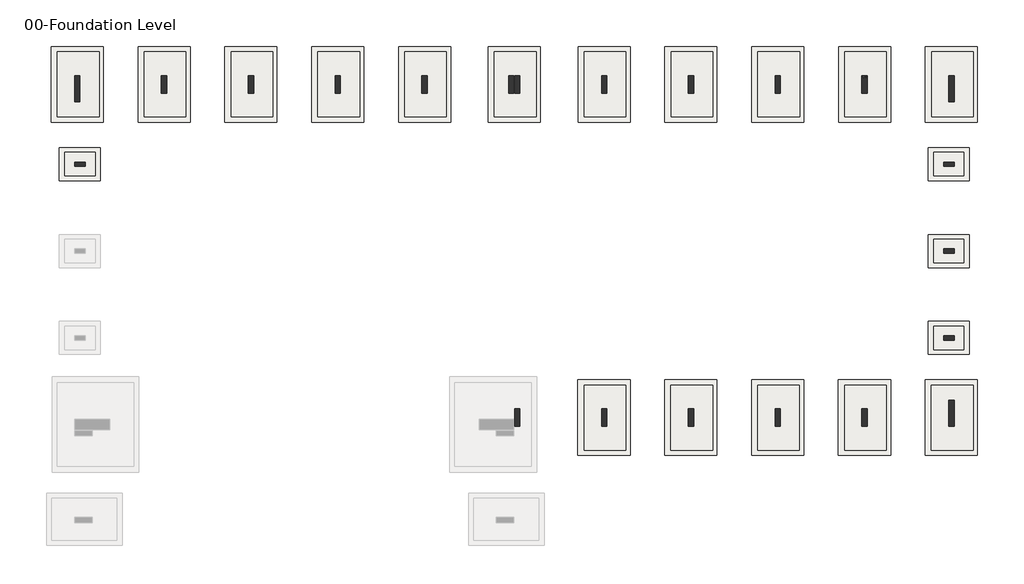
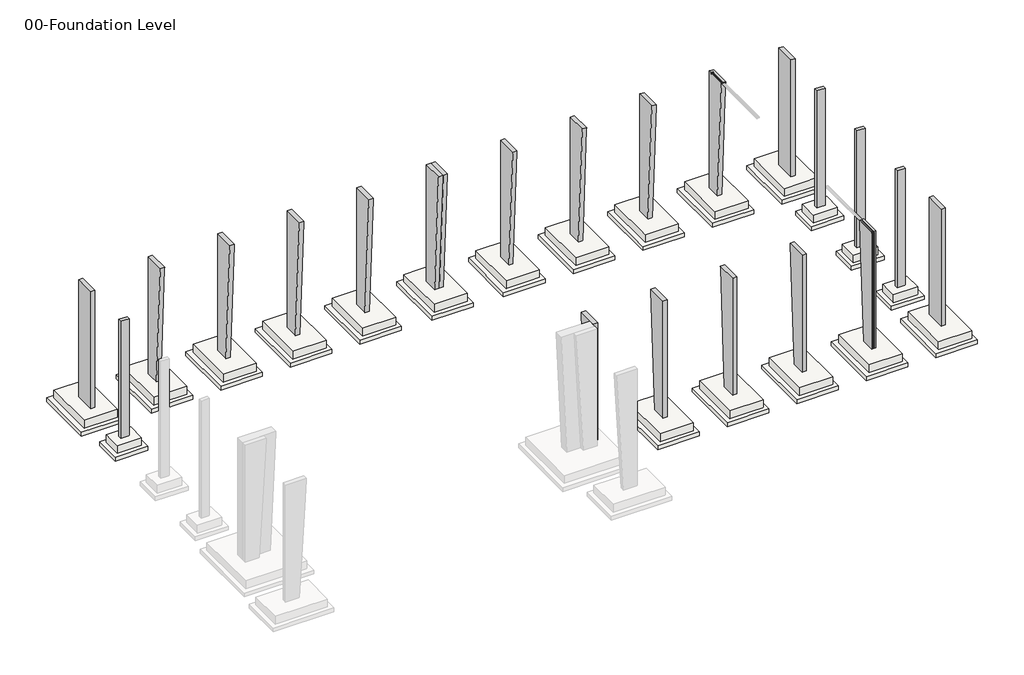
# One storey, part 3 of 4: 40 slabs, 22 columns.
"""IFC4 building model written with IfcOpenShell, lengths in millimetres."""

import ifcopenshell
import ifcopenshell.guid

model = None  # the IFC model being written
_history = None  # IfcOwnerHistory: only IFC2X3 demands one
_inside = {}  # id of a spatial element -> (the spatial element, [elements in it])
_under = {}  # id of a project, library or spatial element -> (it, [spatial elements below it])
_declared = {}  # id of a project -> (the project, [libraries it declares])
_typed = {}  # id of a type object -> (the type object, [elements of that type])
_made_of = {}  # id of a material, layer set ... -> (it, [elements and type objects made of it])


def new_model(schema):
    """Start an empty IFC model of exactly this schema.

    Asked for "IFC4X3", IfcOpenShell would pick the latest addendum, in which some entities
    have other attributes; the version numbers below select the first issue.
    IFC2X3 requires an IfcOwnerHistory on every rooted entity: one is made here for all.
    """
    global model, _history
    if schema == "IFC4X3":
        model = ifcopenshell.file(schema_version=(4, 3, 0, 0))
    else:
        model = ifcopenshell.file(schema=schema)
    _inside.clear()
    _under.clear()
    _declared.clear()
    _typed.clear()
    _made_of.clear()
    _history = None
    if model.schema == "IFC2X3":
        org = make("IfcOrganization", Name="unknown")
        user = make(
            "IfcPersonAndOrganization",
            ThePerson=make("IfcPerson", FamilyName="unknown"),
            TheOrganization=org,
        )
        app = make(
            "IfcApplication",
            ApplicationDeveloper=org,
            Version="unknown",
            ApplicationFullName="unknown",
            ApplicationIdentifier="unknown",
        )
        _history = make(
            "IfcOwnerHistory",
            OwningUser=user,
            OwningApplication=app,
            ChangeAction="ADDED",
            CreationDate=0,
        )
    return model


def make(cls, **values):
    """One entity of the class cls with the attributes given. An attribute that is None is left unset."""
    return model.create_entity(
        cls, **{name: value for name, value in values.items() if value is not None}
    )


def rooted(cls, **values):
    """An entity with a GlobalId (a new one), such as an element, a storey or a relation."""
    return make(cls, GlobalId=ifcopenshell.guid.new(), OwnerHistory=_history, **values)


def si_unit(unit_type, name, prefix=None):
    """IfcSIUnit, for example si_unit("LENGTHUNIT", "METRE", prefix="MILLI")."""
    return make("IfcSIUnit", UnitType=unit_type, Prefix=prefix, Name=name)


def assignment(units):
    """IfcUnitAssignment: the units of a project."""
    return None if units is None else make("IfcUnitAssignment", Units=units)


def point(xyz):
    """IfcCartesianPoint."""
    return None if xyz is None else make("IfcCartesianPoint", Coordinates=xyz)


def direction(xyz):
    """IfcDirection."""
    return None if xyz is None else make("IfcDirection", DirectionRatios=xyz)


def frame(location, z_axis=None, x_axis=None):
    """IfcAxis2Placement3D, a coordinate frame: its origin and axes. An axis left out is left unset."""
    return make(
        "IfcAxis2Placement3D",
        Location=point(location),
        Axis=direction(z_axis),
        RefDirection=direction(x_axis),
    )


def origin():
    """The frame at (0, 0, 0) with its axes left unset."""
    return frame((0.0, 0.0, 0.0))


def place(relative_to, where):
    """IfcLocalPlacement: puts the frame where relative to a parent placement (None: the world)."""
    return make(
        "IfcLocalPlacement", PlacementRelTo=relative_to, RelativePlacement=where
    )


def context(
    kind, dimensions, precision=None, world=None, true_north=None, identifier=None
):
    """IfcGeometricRepresentationContext, for example the 3D "Model" context."""
    return make(
        "IfcGeometricRepresentationContext",
        ContextIdentifier=identifier,
        ContextType=kind,
        CoordinateSpaceDimension=dimensions,
        Precision=precision,
        WorldCoordinateSystem=world,
        TrueNorth=true_north,
    )


def project(units=None, contexts=None):
    """IfcProject with its units and contexts."""
    return rooted(
        "IfcProject",
        Name="project",
        RepresentationContexts=contexts,
        UnitsInContext=assignment(units),
    )


def spatial(cls, under=None, at=None, **own):
    """A site, building, storey or space (cls), placed at a placement, below another one or the project."""
    s = rooted(cls, ObjectPlacement=at, **own)
    if under is not None:
        _under.setdefault(under.id(), (under, []))[1].append(s)
    return s


def polyline(points):
    """IfcPolyline through the points."""
    return make("IfcPolyline", Points=[point(p) for p in points])


def outline(outer, holes=None, kind="AREA"):
    """IfcArbitraryClosedProfileDef: a profile drawn as a closed curve; with holes, ...WithVoids."""
    if holes is None:
        return make("IfcArbitraryClosedProfileDef", ProfileType=kind, OuterCurve=outer)
    return make(
        "IfcArbitraryProfileDefWithVoids",
        ProfileType=kind,
        OuterCurve=outer,
        InnerCurves=holes,
    )


def extrude(swept, where, along, depth):
    """IfcExtrudedAreaSolid: the profile swept, set in the frame where, extruded along a direction by depth."""
    return make(
        "IfcExtrudedAreaSolid",
        SweptArea=swept,
        Position=where,
        ExtrudedDirection=direction(along),
        Depth=depth,
    )


def faces_of(points, faces, orient=None, outer=None):
    """IfcFace entities. A face is a list of loops; a loop is a list of indices into points, from 0.

    orient and outer hold one flag for each loop. By default every Orientation is true, the
    first loop of a face is its IfcFaceOuterBound and the others are IfcFaceBound.
    """
    made = []
    for i, loops in enumerate(faces):
        bounds = []
        for j, loop in enumerate(loops):
            is_outer = j == 0 if outer is None else outer[i][j]
            bounds.append(
                make(
                    "IfcFaceOuterBound" if is_outer else "IfcFaceBound",
                    Bound=make("IfcPolyLoop", Polygon=[points[k] for k in loop]),
                    Orientation=True if orient is None else orient[i][j],
                )
            )
        made.append(make("IfcFace", Bounds=bounds))
    return made


def faceted_brep(points, faces, orient=None, outer=None, voids=None):
    """IfcFacetedBrep: a solid bounded by flat faces; with voids (closed shells), ...WithVoids."""
    shared = [point(p) for p in points]
    hull = make("IfcClosedShell", CfsFaces=faces_of(shared, faces, orient, outer))
    if voids is None:
        return make("IfcFacetedBrep", Outer=hull)
    return make(
        "IfcFacetedBrepWithVoids",
        Outer=hull,
        Voids=[
            make(cls, CfsFaces=faces_of(shared, fs, o, b)) for cls, fs, o, b in voids
        ],
    )


def shape(context_of_items, identifier, shape_type, items):
    """IfcShapeRepresentation: the items that make up one representation, for example the "Body"."""
    return make(
        "IfcShapeRepresentation",
        ContextOfItems=context_of_items,
        RepresentationIdentifier=identifier,
        RepresentationType=shape_type,
        Items=items,
    )


def made_of(thing, what):
    """Note that an element or type object is made of a material, layer set ...; save() writes the relation."""
    if what is not None:
        _made_of.setdefault(what.id(), (what, []))[1].append(thing)
    return thing


def element(
    cls,
    number,
    at=None,
    inside=None,
    cuts=None,
    type_object=None,
    material=None,
    context=None,
    identifier="Body",
    shape_type=None,
    held_by="IfcProductDefinitionShape",
    body=None,
    shapes=None,
    **own,
):
    """One element of the class cls, such as IfcWall. Its Tag is "e" and its number.

    at: its placement. inside: the storey or other place that contains it. cuts: it is an
    opening in that element (IfcRelVoidsElement). A single representation is given by context,
    identifier, shape_type and body (its items); several are given by shapes. held_by: the class
    of the entity that holds the representations. save() writes the other relations.
    """
    e = rooted(cls, Tag="e%d" % number, ObjectPlacement=at, **own)
    if body is not None:
        shapes = [shape(context, identifier, shape_type, body)]
    if shapes is not None:
        e.Representation = make(held_by, Representations=shapes)
    if inside is not None:
        _inside.setdefault(inside.id(), (inside, []))[1].append(e)
    if cuts is not None:
        rooted(
            "IfcRelVoidsElement", RelatingBuildingElement=cuts, RelatedOpeningElement=e
        )
    if type_object is not None:
        _typed.setdefault(type_object.id(), (type_object, []))[1].append(e)
    return made_of(e, material)


def aggregate(whole, parts):
    """IfcRelAggregates: a whole, such as a stair, and the parts it consists of."""
    return rooted("IfcRelAggregates", RelatingObject=whole, RelatedObjects=parts)


def save(model, path):
    """Write the relations noted so far, then the file.

    IfcRelAggregates (storeys below a building ...), IfcRelContainedInSpatialStructure (elements
    in a storey), IfcRelDefinesByType, IfcRelAssociatesMaterial and IfcRelDeclares: one each for
    every whole, place, type object, material and project.
    """
    for whole, parts in _under.values():
        aggregate(whole, parts)
    for where, things in _inside.values():
        rooted(
            "IfcRelContainedInSpatialStructure",
            RelatedElements=things,
            RelatingStructure=where,
        )
    for kind, things in _typed.values():
        rooted("IfcRelDefinesByType", RelatedObjects=things, RelatingType=kind)
    for what, things in _made_of.values():
        rooted("IfcRelAssociatesMaterial", RelatedObjects=things, RelatingMaterial=what)
    for by, libraries in _declared.values():
        rooted("IfcRelDeclares", RelatingContext=by, RelatedDefinitions=libraries)
    model.write(path)


model = new_model("IFC4")

# Units and contexts
model_context = context("Model", 3, world=origin())
ifc_project = project(units=[si_unit("LENGTHUNIT", "METRE", prefix="MILLI")], contexts=[model_context])

# Site, building, storey
site = spatial("IfcSite", under=ifc_project)
building = spatial("IfcBuilding", under=site)
storey = spatial("IfcBuildingStorey", under=building, Name="00-Foundation Level", Elevation=-2000.0)

# Columns
placement = place(None, origin())
element("IfcColumn", 1, ObjectType="Frame Col.2 : 1500x300", at=placement, inside=storey, context=model_context, shape_type="Brep", body=[
    faceted_brep([(50823.2245514, 70079.74482, -1100.0), (50823.2245514, 71079.74482, -1100.0), (50823.2245514, 71079.74482, 7680.0), (50823.2245514, 71079.74482, 7800.0), (50823.2245514, 69579.74482, 7800.0), (50823.2245514, 69586.4863931, 7680.0), (50523.2245514, 69579.74482, 7800.0), (50523.2245514, 69586.4863931, 7680.0), (50523.2245514, 70079.74482, -1100.0), (50523.2245514, 71079.74482, -1100.0), (50523.2245514, 71079.74482, 7800.0)], [[[0, 1, 2, 3, 4, 5]], [[0, 5, 4, 6, 7, 8]], [[9, 8, 7, 6, 10]], [[3, 2, 1, 9, 10]], [[1, 0, 8, 9]], [[4, 3, 10, 6]]]),
])
element("IfcColumn", 2, ObjectType="Frame Col.2 : 1500x300", at=placement, inside=storey, context=model_context, shape_type="Brep", body=[
    faceted_brep([(30483.2245515, 70079.74482, -1100.0), (30483.2245515, 71079.74482, -1100.0), (30483.2245515, 71079.74482, 7680.0), (30483.2245515, 71079.74482, 7800.0), (30483.2245515, 69579.74482, 7800.0), (30483.2245515, 69586.4863931, 7680.0), (30183.2245515, 69579.74482, 7800.0), (30183.2245515, 69586.4863931, 7680.0), (30183.2245515, 70079.74482, -1100.0), (30183.2245515, 71079.74482, -1100.0), (30183.2245515, 71079.74482, 7800.0), (30183.2245515, 71079.74482, 7680.0)], [[[0, 1, 2, 3, 4, 5]], [[0, 5, 4, 6, 7, 8]], [[9, 8, 7, 6, 10, 11]], [[3, 2, 1, 9, 11, 10]], [[1, 0, 8, 9]], [[4, 3, 10, 6]]]),
])
element("IfcColumn", 3, ObjectType="Frame Col.2 : 1500x300", at=placement, inside=storey, context=model_context, shape_type="Brep", body=[
    faceted_brep([(50523.2245514, 51879.7448203, -1100.0), (50523.2245514, 50879.7448203, -1100.0), (50523.2245514, 50879.7448203, 7800.0), (50523.2245514, 52379.7448203, 7800.0), (50523.2245514, 52373.0032473, 7680.0), (50823.2245514, 52379.7448203, 7800.0), (50823.2245514, 52373.0032473, 7680.0), (50823.2245514, 51879.7448203, -1100.0), (50823.2245514, 50879.7448203, -1100.0), (50823.2245514, 50879.7448203, 7800.0), (50823.2245514, 50879.7448203, 7680.0)], [[[0, 1, 2, 3, 4]], [[0, 4, 3, 5, 6, 7]], [[8, 7, 6, 5, 9, 10]], [[2, 1, 8, 10, 9]], [[1, 0, 7, 8]], [[3, 2, 9, 5]]]),
])
element("IfcColumn", 4, ObjectType="Frame Col.2 : 1500x300", at=placement, inside=storey, context=model_context, shape_type="Brep", body=[
    faceted_brep([(35483.2245515, 70079.74482, -1100.0), (35483.2245515, 71079.74482, -1100.0), (35483.2245515, 71079.74482, 7680.0), (35483.2245515, 71079.74482, 7800.0), (35483.2245515, 69579.74482, 7800.0), (35483.2245515, 69586.4863931, 7680.0), (35183.2245515, 69579.74482, 7800.0), (35183.2245515, 69586.4863931, 7680.0), (35183.2245515, 70079.74482, -1100.0), (35183.2245515, 71079.74482, -1100.0), (35183.2245515, 71079.74482, 7800.0), (35183.2245515, 71079.74482, 7680.0)], [[[0, 1, 2, 3, 4, 5]], [[0, 5, 4, 6, 7, 8]], [[9, 8, 7, 6, 10, 11]], [[3, 2, 1, 9, 11, 10]], [[1, 0, 8, 9]], [[4, 3, 10, 6]]]),
])
element("IfcColumn", 5, ObjectType="Frame Col.2 : 1500x300", at=placement, inside=storey, context=model_context, shape_type="Brep", body=[
    faceted_brep([(40483.2245515, 70079.74482, -1100.0), (40483.2245515, 71079.74482, -1100.0), (40483.2245515, 71079.74482, 7680.0), (40483.2245515, 71079.74482, 7800.0), (40483.2245515, 69579.74482, 7800.0), (40483.2245515, 69586.4863931, 7680.0), (40183.2245515, 69579.74482, 7800.0), (40183.2245515, 69586.4863931, 7680.0), (40183.2245515, 70079.74482, -1100.0), (40183.2245515, 71079.74482, -1100.0), (40183.2245515, 71079.74482, 7800.0), (40183.2245515, 71079.74482, 7680.0)], [[[0, 1, 2, 3, 4, 5]], [[0, 5, 4, 6, 7, 8]], [[9, 8, 7, 6, 10, 11]], [[3, 2, 1, 9, 11, 10]], [[1, 0, 8, 9]], [[4, 3, 10, 6]]]),
])
element("IfcColumn", 6, ObjectType="Frame Col.2 : 1500x300", at=placement, inside=storey, context=model_context, shape_type="Brep", body=[
    faceted_brep([(45483.2245515, 70079.74482, -1100.0), (45483.2245515, 71079.74482, -1100.0), (45483.2245515, 71079.74482, 7680.0), (45483.2245515, 71079.74482, 7800.0), (45483.2245515, 69579.74482, 7800.0), (45483.2245515, 69586.4863931, 7680.0), (45183.2245515, 69579.74482, 7800.0), (45183.2245515, 69586.4863931, 7680.0), (45183.2245515, 70079.74482, -1100.0), (45183.2245515, 71079.74482, -1100.0), (45183.2245515, 71079.74482, 7800.0), (45183.2245515, 71079.74482, 7680.0)], [[[0, 1, 2, 3, 4, 5]], [[0, 5, 4, 6, 7, 8]], [[9, 8, 7, 6, 10, 11]], [[3, 2, 1, 9, 11, 10]], [[1, 0, 8, 9]], [[4, 3, 10, 6]]]),
])
element("IfcColumn", 7, ObjectType="Frame Col.2 : 1500x300", at=placement, inside=storey, context=model_context, shape_type="Brep", body=[
    faceted_brep([(50483.2245514, 70079.74482, -1100.0), (50483.2245514, 71079.74482, -1100.0), (50483.2245514, 71079.74482, 7800.0), (50483.2245514, 69579.74482, 7800.0), (50483.2245514, 69586.4863931, 7680.0), (50183.2245514, 69579.74482, 7800.0), (50183.2245514, 69586.4863931, 7680.0), (50183.2245514, 70079.74482, -1100.0), (50183.2245514, 71079.74482, -1100.0), (50183.2245514, 71079.74482, 7800.0), (50183.2245514, 71079.74482, 7680.0)], [[[0, 1, 2, 3, 4]], [[0, 4, 3, 5, 6, 7]], [[8, 7, 6, 5, 9, 10]], [[2, 1, 8, 10, 9]], [[1, 0, 7, 8]], [[3, 2, 9, 5]]]),
])
element("IfcColumn", 8, ObjectType="Frame Col.2 : 1500x300", at=placement, inside=storey, context=model_context, shape_type="Brep", body=[
    faceted_brep([(55823.2245516, 70079.74482, -1100.0), (55823.2245516, 71079.74482, -1100.0), (55823.2245516, 71079.74482, 7680.0), (55823.2245516, 71079.74482, 7800.0), (55823.2245516, 69579.74482, 7800.0), (55823.2245516, 69586.4863931, 7680.0), (55523.2245516, 69579.74482, 7800.0), (55523.2245516, 69586.4863931, 7680.0), (55523.2245516, 70079.74482, -1100.0), (55523.2245516, 71079.74482, -1100.0), (55523.2245516, 71079.74482, 7800.0), (55523.2245516, 71079.74482, 7680.0)], [[[0, 1, 2, 3, 4, 5]], [[0, 5, 4, 6, 7, 8]], [[9, 8, 7, 6, 10, 11]], [[3, 2, 1, 9, 11, 10]], [[1, 0, 8, 9]], [[4, 3, 10, 6]]]),
])
element("IfcColumn", 9, ObjectType="Frame Col.2 : 1500x300", at=placement, inside=storey, context=model_context, shape_type="Brep", body=[
    faceted_brep([(55523.2245516, 51879.7448203, -1100.0), (55523.2245516, 50879.7448203, -1100.0), (55523.2245516, 50879.7448203, 7680.0), (55523.2245516, 50879.7448203, 7800.0), (55523.2245516, 52379.7448203, 7800.0), (55523.2245516, 52373.0032473, 7680.0), (55823.2245516, 52379.7448203, 7800.0), (55823.2245516, 52373.0032473, 7680.0), (55823.2245516, 51879.7448203, -1100.0), (55823.2245516, 50879.7448203, -1100.0), (55823.2245516, 50879.7448203, 7800.0), (55823.2245516, 50879.7448203, 7680.0)], [[[0, 1, 2, 3, 4, 5]], [[0, 5, 4, 6, 7, 8]], [[9, 8, 7, 6, 10, 11]], [[3, 2, 1, 9, 11, 10]], [[1, 0, 8, 9]], [[4, 3, 10, 6]]]),
])
element("IfcColumn", 10, ObjectType="Frame Col.2 : 1500x300", at=placement, inside=storey, context=model_context, shape_type="Brep", body=[
    faceted_brep([(60823.2245516, 70079.74482, -1100.0), (60823.2245516, 71079.74482, -1100.0), (60823.2245516, 71079.74482, 7680.0), (60823.2245516, 71079.74482, 7800.0), (60823.2245516, 69579.74482, 7800.0), (60823.2245516, 69586.4863931, 7680.0), (60523.2245516, 69579.74482, 7800.0), (60523.2245516, 69586.4863931, 7680.0), (60523.2245516, 70079.74482, -1100.0), (60523.2245516, 71079.74482, -1100.0), (60523.2245516, 71079.74482, 7800.0), (60523.2245516, 71079.74482, 7680.0)], [[[0, 1, 2, 3, 4, 5]], [[0, 5, 4, 6, 7, 8]], [[9, 8, 7, 6, 10, 11]], [[3, 2, 1, 9, 11, 10]], [[1, 0, 8, 9]], [[4, 3, 10, 6]]]),
])
element("IfcColumn", 11, ObjectType="Frame Col.2 : 1500x300", at=placement, inside=storey, context=model_context, shape_type="Brep", body=[
    faceted_brep([(60523.2245516, 51879.7448203, -1100.0), (60523.2245516, 50879.7448203, -1100.0), (60523.2245516, 50879.7448203, 7680.0), (60523.2245516, 50879.7448203, 7800.0), (60523.2245516, 52379.7448203, 7800.0), (60523.2245516, 52373.0032473, 7680.0), (60823.2245516, 52379.7448203, 7800.0), (60823.2245516, 52373.0032473, 7680.0), (60823.2245516, 51879.7448203, -1100.0), (60823.2245516, 50879.7448203, -1100.0), (60823.2245516, 50879.7448203, 7800.0), (60823.2245516, 50879.7448203, 7680.0)], [[[0, 1, 2, 3, 4, 5]], [[0, 5, 4, 6, 7, 8]], [[9, 8, 7, 6, 10, 11]], [[3, 2, 1, 9, 11, 10]], [[1, 0, 8, 9]], [[4, 3, 10, 6]]]),
])
element("IfcColumn", 12, ObjectType="Frame Col.2 : 1500x300", at=placement, inside=storey, context=model_context, shape_type="Brep", body=[
    faceted_brep([(65823.2245516, 70079.74482, -1100.0), (65823.2245516, 71079.74482, -1100.0), (65823.2245516, 71079.74482, 7680.0), (65823.2245516, 71079.74482, 7800.0), (65823.2245516, 69579.74482, 7800.0), (65823.2245516, 69586.4863931, 7680.0), (65523.2245516, 69579.74482, 7800.0), (65523.2245516, 69586.4863931, 7680.0), (65523.2245516, 70079.74482, -1100.0), (65523.2245516, 71079.74482, -1100.0), (65523.2245516, 71079.74482, 7800.0), (65523.2245516, 71079.74482, 7680.0)], [[[0, 1, 2, 3, 4, 5]], [[0, 5, 4, 6, 7, 8]], [[9, 8, 7, 6, 10, 11]], [[3, 2, 1, 9, 11, 10]], [[1, 0, 8, 9]], [[4, 3, 10, 6]]]),
])
element("IfcColumn", 13, ObjectType="Frame Col.2 : 1500x300", at=placement, inside=storey, context=model_context, shape_type="Brep", body=[
    faceted_brep([(65523.2245516, 51879.7448203, -1100.0), (65523.2245516, 50879.7448203, -1100.0), (65523.2245516, 50879.7448203, 7680.0), (65523.2245516, 50879.7448203, 7800.0), (65523.2245516, 52379.7448203, 7800.0), (65523.2245516, 52373.0032473, 7680.0), (65823.2245516, 52379.7448203, 7800.0), (65823.2245516, 52373.0032473, 7680.0), (65823.2245516, 51879.7448203, -1100.0), (65823.2245516, 50879.7448203, -1100.0), (65823.2245516, 50879.7448203, 7800.0), (65823.2245516, 50879.7448203, 7680.0)], [[[0, 1, 2, 3, 4, 5]], [[0, 5, 4, 6, 7, 8]], [[9, 8, 7, 6, 10, 11]], [[3, 2, 1, 9, 11, 10]], [[1, 0, 8, 9]], [[4, 3, 10, 6]]]),
])
element("IfcColumn", 14, ObjectType="Frame Col.2 : 1500x300", at=placement, inside=storey, context=model_context, shape_type="Brep", body=[
    faceted_brep([(70823.2245516, 70079.74482, -1100.0), (70823.2245516, 71079.74482, -1100.0), (70823.2245516, 71079.74482, 7680.0), (70823.2245516, 71079.74482, 7800.0), (70823.2245516, 69579.74482, 7800.0), (70823.2245516, 69586.4863931, 7680.0), (70823.2245516, 69664.0144829, 6300.0), (70523.2245516, 69579.74482, 7800.0), (70523.2245516, 69586.4863931, 7680.0), (70523.2245516, 69664.0144829, 6300.0), (70523.2245516, 70079.74482, -1100.0), (70523.2245516, 71079.74482, -1100.0), (70523.2245516, 71079.74482, 7800.0), (70523.2245516, 71079.74482, 7680.0)], [[[0, 1, 2, 3, 4, 5, 6]], [[0, 6, 5, 4, 7, 8, 9, 10]], [[11, 10, 9, 8, 7, 12, 13]], [[3, 2, 1, 11, 13, 12]], [[1, 0, 10, 11]], [[4, 3, 12, 7]]]),
])
element("IfcColumn", 15, ObjectType="Frame Col.2 : 1500x300", at=placement, inside=storey, context=model_context, shape_type="Brep", body=[
    faceted_brep([(70523.2245516, 51879.7448203, -1100.0), (70523.2245516, 50879.7448203, -1100.0), (70523.2245516, 50879.7448203, 7680.0), (70523.2245516, 50879.7448203, 7800.0), (70523.2245516, 52379.7448203, 7800.0), (70523.2245516, 52373.0032473, 7680.0), (70523.2245516, 52295.4751574, 6300.0), (70823.2245516, 52379.7448203, 7800.0), (70823.2245516, 52373.0032473, 7680.0), (70823.2245516, 52295.4751574, 6300.0), (70823.2245516, 51879.7448203, -1100.0), (70823.2245516, 50879.7448203, -1100.0), (70823.2245516, 50879.7448203, 7800.0), (70823.2245516, 50879.7448203, 7680.0)], [[[0, 1, 2, 3, 4, 5, 6]], [[0, 6, 5, 4, 7, 8, 9, 10]], [[11, 10, 9, 8, 7, 12, 13]], [[3, 2, 1, 11, 13, 12]], [[1, 0, 10, 11]], [[4, 3, 12, 7]]]),
])
element("IfcColumn", 16, ObjectType="M_Concrete-Rectangular-Column : 250 x 600mm", at=placement, inside=storey, context=model_context, shape_type="Brep", body=[
    faceted_brep([(75223.2245516, 66104.9999988, -1100.0), (75823.2245516, 66104.9999988, -1100.0), (75823.2245516, 65854.9999988, -1100.0), (75223.2245516, 65854.9999988, -1100.0), (75223.2245516, 66104.9999988, 7680.0), (75223.2245516, 66104.9999988, 7800.0), (75823.2245516, 66104.9999988, 7800.0), (75823.2245516, 66104.9999988, 7680.0), (75823.2245516, 65854.9999988, 7800.0), (75823.2245516, 65854.9999988, 7680.0), (75223.2245516, 65854.9999988, 7800.0), (75223.2245516, 65854.9999988, 7680.0)], [[[0, 1, 2, 3]], [[1, 0, 4, 5, 6, 7]], [[2, 1, 7, 6, 8, 9]], [[3, 2, 9, 8, 10, 11]], [[0, 3, 11, 10, 5, 4]], [[6, 5, 10, 8]]]),
])
element("IfcColumn", 17, ObjectType="M_Concrete-Rectangular-Column : 250 x 600mm", at=placement, inside=storey, context=model_context, shape_type="Brep", body=[
    faceted_brep([(75223.2245516, 61104.74482, -1100.0), (75823.2245516, 61104.74482, -1100.0), (75823.2245516, 60854.74482, -1100.0), (75223.2245516, 60854.74482, -1100.0), (75223.2245516, 61104.74482, 7680.0), (75223.2245516, 61104.74482, 7800.0), (75823.2245516, 61104.74482, 7800.0), (75823.2245516, 61104.74482, 7680.0), (75823.2245516, 60854.74482, 7800.0), (75823.2245516, 60854.74482, 7680.0), (75223.2245516, 60854.74482, 7800.0), (75223.2245516, 60854.74482, 7680.0)], [[[0, 1, 2, 3]], [[1, 0, 4, 5, 6, 7]], [[2, 1, 7, 6, 8, 9]], [[3, 2, 9, 8, 10, 11]], [[0, 3, 11, 10, 5, 4]], [[6, 5, 10, 8]]]),
])
element("IfcColumn", 18, ObjectType="M_Concrete-Rectangular-Column : 250 x 600mm", at=placement, inside=storey, context=model_context, shape_type="Brep", body=[
    faceted_brep([(75223.2245516, 56104.9999988, -1100.0), (75823.2245516, 56104.9999988, -1100.0), (75823.2245516, 55854.9999988, -1100.0), (75223.2245516, 55854.9999988, -1100.0), (75223.2245516, 56104.9999988, 7680.0), (75223.2245516, 56104.9999988, 7800.0), (75823.2245516, 56104.9999988, 7800.0), (75823.2245516, 56104.9999988, 7680.0), (75823.2245516, 55854.9999988, 7800.0), (75823.2245516, 55854.9999988, 7680.0), (75223.2245516, 55854.9999988, 7800.0), (75223.2245516, 55854.9999988, 7680.0)], [[[0, 1, 2, 3]], [[1, 0, 4, 5, 6, 7]], [[2, 1, 7, 6, 8, 9]], [[3, 2, 9, 8, 10, 11]], [[0, 3, 11, 10, 5, 4]], [[6, 5, 10, 8]]]),
])
element("IfcColumn", 19, ObjectType="M_Concrete-Rectangular-Column : 250 x 600mm", at=placement, inside=storey, context=model_context, shape_type="Brep", body=[
    faceted_brep([(25183.2245516, 66104.9999988, -1100.0), (25783.2245516, 66104.9999988, -1100.0), (25783.2245516, 65854.9999988, -1100.0), (25183.2245516, 65854.9999988, -1100.0), (25183.2245516, 66104.9999988, 7680.0), (25183.2245516, 66104.9999988, 7800.0), (25783.2245516, 66104.9999988, 7800.0), (25783.2245516, 66104.9999988, 7680.0), (25183.2245516, 65854.9999988, 7680.0), (25183.2245516, 65854.9999988, 7800.0), (25783.2245516, 65854.9999988, 7680.0), (25783.2245516, 65854.9999988, 7800.0)], [[[0, 1, 2, 3]], [[1, 0, 4, 5, 6, 7]], [[0, 3, 8, 9, 5, 4]], [[3, 2, 10, 11, 9, 8]], [[2, 1, 7, 6, 11, 10]], [[6, 5, 9, 11]]]),
])
element("IfcColumn", 20, ObjectType="M_Concrete-Rectangular-Column : 300 x 1500mm", at=placement, inside=storey, context=model_context, shape_type="Brep", body=[
    faceted_brep([(75823.2245516, 71079.74482, -1100.0), (75823.2245516, 69579.74482, -1100.0), (75523.2245516, 69579.74482, -1100.0), (75523.2245516, 71079.74482, -1100.0), (75823.2245516, 71079.74482, 7800.0), (75823.2245516, 69579.74482, 7800.0), (75823.2245516, 69579.74482, 7680.0), (75523.2245516, 69579.74482, 7800.0), (75523.2245516, 69579.74482, 7680.0), (75523.2245516, 71079.74482, 7800.0), (75523.2245516, 71079.74482, 7680.0)], [[[0, 1, 2, 3]], [[1, 0, 4, 5, 6]], [[2, 1, 6, 5, 7, 8]], [[3, 2, 8, 7, 9, 10]], [[0, 3, 10, 9, 4]], [[5, 4, 9, 7]]]),
])
element("IfcColumn", 21, ObjectType="M_Concrete-Rectangular-Column : 300 x 1500mm", at=placement, inside=storey, context=model_context, shape_type="Brep", body=[
    faceted_brep([(75823.2245516, 52379.7448203, -1100.0), (75823.2245516, 50879.7448203, -1100.0), (75523.2245516, 50879.7448203, -1100.0), (75523.2245516, 52379.7448203, -1100.0), (75823.2245516, 52379.7448203, 7680.0), (75823.2245516, 52379.7448203, 7800.0), (75823.2245516, 50879.7448203, 7800.0), (75523.2245516, 50879.7448203, 7800.0), (75523.2245516, 50879.7448203, 7680.0), (75523.2245516, 52379.7448203, 7800.0), (75523.2245516, 52379.7448203, 7680.0)], [[[0, 1, 2, 3]], [[1, 0, 4, 5, 6]], [[2, 1, 6, 7, 8]], [[3, 2, 8, 7, 9, 10]], [[0, 3, 10, 9, 5, 4]], [[6, 5, 9, 7]]]),
])
element("IfcColumn", 22, ObjectType="M_Concrete-Rectangular-Column : 300 x 1500mm", at=placement, inside=storey, context=model_context, shape_type="Brep", body=[
    faceted_brep([(25183.2245516, 69579.74482, -1100.0), (25183.2245516, 71079.74482, -1100.0), (25483.2245516, 71079.74482, -1100.0), (25483.2245516, 69579.74482, -1100.0), (25183.2245516, 69579.74482, 7680.0), (25183.2245516, 69579.74482, 7800.0), (25183.2245516, 71079.74482, 7800.0), (25483.2245516, 69579.74482, 7680.0), (25483.2245516, 69579.74482, 7800.0), (25483.2245516, 71079.74482, 7680.0), (25483.2245516, 71079.74482, 7800.0)], [[[0, 1, 2, 3]], [[1, 0, 4, 5, 6]], [[0, 3, 7, 8, 5, 4]], [[3, 2, 9, 10, 8, 7]], [[2, 1, 6, 10, 9]], [[6, 5, 8, 10]]]),
])

# Slabs
element("IfcSlab", 23, ObjectType="M_Footing-Rectangular : PC 2-2350 x 1900 x 300mm", at=placement, inside=storey, context=model_context, shape_type="SweptSolid", body=[
    extrude(outline(polyline([(76698.2245516, 66929.9999988), (76698.2245516, 65029.9999988), (74348.2245516, 65029.9999988), (74348.2245516, 66929.9999988), (76698.2245516, 66929.9999988)])), frame((0.0, 0.0, -2000.0), z_axis=(0.0, 0.0, 1.0), x_axis=(1.0, 0.0, 0.0)), (0.0, 0.0, 1.0), 300.0),
])
element("IfcSlab", 24, ObjectType="M_Footing-Rectangular : PC 2-2350 x 1900 x 300mm", at=placement, inside=storey, context=model_context, shape_type="SweptSolid", body=[
    extrude(outline(polyline([(76698.2245516, 61929.9999988), (76698.2245516, 60029.9999988), (74348.2245516, 60029.9999988), (74348.2245516, 61929.9999988), (76698.2245516, 61929.9999988)])), frame((0.0, 0.0, -2000.0), z_axis=(0.0, 0.0, 1.0), x_axis=(1.0, 0.0, 0.0)), (0.0, 0.0, 1.0), 300.0),
])
element("IfcSlab", 25, ObjectType="M_Footing-Rectangular : PC 2-2350 x 1900 x 300mm", at=placement, inside=storey, context=model_context, shape_type="SweptSolid", body=[
    extrude(outline(polyline([(76698.2245516, 56929.9999988), (76698.2245516, 55029.9999988), (74348.2245516, 55029.9999988), (74348.2245516, 56929.9999988), (76698.2245516, 56929.9999988)])), frame((0.0, 0.0, -2000.0), z_axis=(0.0, 0.0, 1.0), x_axis=(1.0, 0.0, 0.0)), (0.0, 0.0, 1.0), 300.0),
])
element("IfcSlab", 26, ObjectType="M_Footing-Rectangular : PC 2-2350 x 1900 x 300mm", at=placement, inside=storey, context=model_context, shape_type="SweptSolid", body=[
    extrude(outline(polyline([(26658.2245516, 66929.9999988), (26658.2245516, 65029.9999988), (24308.2245516, 65029.9999988), (24308.2245516, 66929.9999988), (26658.2245516, 66929.9999988)])), frame((0.0, 0.0, -2000.0), z_axis=(0.0, 0.0, 1.0), x_axis=(1.0, 0.0, 0.0)), (0.0, 0.0, 1.0), 300.0),
])
element("IfcSlab", 27, ObjectType="M_Footing-Rectangular : PC-4350 x 3000 x 300mm", at=placement, inside=storey, context=model_context, shape_type="SweptSolid", body=[
    extrude(outline(polyline([(77173.2245516, 72754.74482), (77173.2245516, 68404.74482), (74173.2245516, 68404.74482), (74173.2245516, 72754.74482), (77173.2245516, 72754.74482)])), frame((0.0, 0.0, -2000.0), z_axis=(0.0, 0.0, 1.0), x_axis=(1.0, 0.0, 0.0)), (0.0, 0.0, 1.0), 300.0),
])
element("IfcSlab", 28, ObjectType="M_Footing-Rectangular : PC-4350 x 3000 x 300mm", at=placement, inside=storey, context=model_context, shape_type="SweptSolid", body=[
    extrude(outline(polyline([(77166.9023264, 53554.7448203), (77166.9023264, 49204.7448203), (74166.9023264, 49204.7448203), (74166.9023264, 53554.7448203), (77166.9023264, 53554.7448203)])), frame((0.0, 0.0, -2000.0), z_axis=(0.0, 0.0, 1.0), x_axis=(1.0, 0.0, 0.0)), (0.0, 0.0, 1.0), 300.0),
])
element("IfcSlab", 29, ObjectType="M_Footing-Rectangular : PC-4350 x 3000 x 300mm", at=placement, inside=storey, context=model_context, shape_type="SweptSolid", body=[
    extrude(outline(polyline([(72173.2245516, 72754.74482), (72173.2245516, 68404.74482), (69173.2245516, 68404.74482), (69173.2245516, 72754.74482), (72173.2245516, 72754.74482)])), frame((0.0, 0.0, -2000.0), z_axis=(0.0, 0.0, 1.0), x_axis=(1.0, 0.0, 0.0)), (0.0, 0.0, 1.0), 300.0),
])
element("IfcSlab", 30, ObjectType="M_Footing-Rectangular : PC-4350 x 3000 x 300mm", at=placement, inside=storey, context=model_context, shape_type="SweptSolid", body=[
    extrude(outline(polyline([(72166.9023264, 53554.7448203), (72166.9023264, 49204.7448203), (69166.9023264, 49204.7448203), (69166.9023264, 53554.7448203), (72166.9023264, 53554.7448203)])), frame((0.0, 0.0, -2000.0), z_axis=(0.0, 0.0, 1.0), x_axis=(1.0, 0.0, 0.0)), (0.0, 0.0, 1.0), 300.0),
])
element("IfcSlab", 31, ObjectType="M_Footing-Rectangular : PC-4350 x 3000 x 300mm", at=placement, inside=storey, context=model_context, shape_type="SweptSolid", body=[
    extrude(outline(polyline([(67173.2245516, 72754.74482), (67173.2245516, 68404.74482), (64173.2245516, 68404.74482), (64173.2245516, 72754.74482), (67173.2245516, 72754.74482)])), frame((0.0, 0.0, -2000.0), z_axis=(0.0, 0.0, 1.0), x_axis=(1.0, 0.0, 0.0)), (0.0, 0.0, 1.0), 300.0),
])
element("IfcSlab", 32, ObjectType="M_Footing-Rectangular : PC-4350 x 3000 x 300mm", at=placement, inside=storey, context=model_context, shape_type="SweptSolid", body=[
    extrude(outline(polyline([(67166.9023264, 53554.7448203), (67166.9023264, 49204.7448203), (64166.9023264, 49204.7448203), (64166.9023264, 53554.7448203), (67166.9023264, 53554.7448203)])), frame((0.0, 0.0, -2000.0), z_axis=(0.0, 0.0, 1.0), x_axis=(1.0, 0.0, 0.0)), (0.0, 0.0, 1.0), 300.0),
])
element("IfcSlab", 33, ObjectType="M_Footing-Rectangular : PC-4350 x 3000 x 300mm", at=placement, inside=storey, context=model_context, shape_type="SweptSolid", body=[
    extrude(outline(polyline([(62173.2245516, 72754.74482), (62173.2245516, 68404.74482), (59173.2245516, 68404.74482), (59173.2245516, 72754.74482), (62173.2245516, 72754.74482)])), frame((0.0, 0.0, -2000.0), z_axis=(0.0, 0.0, 1.0), x_axis=(1.0, 0.0, 0.0)), (0.0, 0.0, 1.0), 300.0),
])
element("IfcSlab", 34, ObjectType="M_Footing-Rectangular : PC-4350 x 3000 x 300mm", at=placement, inside=storey, context=model_context, shape_type="SweptSolid", body=[
    extrude(outline(polyline([(62166.9023264, 53554.7448203), (62166.9023264, 49204.7448203), (59166.9023264, 49204.7448203), (59166.9023264, 53554.7448203), (62166.9023264, 53554.7448203)])), frame((0.0, 0.0, -2000.0), z_axis=(0.0, 0.0, 1.0), x_axis=(1.0, 0.0, 0.0)), (0.0, 0.0, 1.0), 300.0),
])
element("IfcSlab", 35, ObjectType="M_Footing-Rectangular : PC-4350 x 3000 x 300mm", at=placement, inside=storey, context=model_context, shape_type="SweptSolid", body=[
    extrude(outline(polyline([(57173.2245516, 72754.74482), (57173.2245516, 68404.74482), (54173.2245516, 68404.74482), (54173.2245516, 72754.74482), (57173.2245516, 72754.74482)])), frame((0.0, 0.0, -2000.0), z_axis=(0.0, 0.0, 1.0), x_axis=(1.0, 0.0, 0.0)), (0.0, 0.0, 1.0), 300.0),
])
element("IfcSlab", 36, ObjectType="M_Footing-Rectangular : PC-4350 x 3000 x 300mm", at=placement, inside=storey, context=model_context, shape_type="SweptSolid", body=[
    extrude(outline(polyline([(57166.9023264, 53554.7448203), (57166.9023264, 49204.7448203), (54166.9023264, 49204.7448203), (54166.9023264, 53554.7448203), (57166.9023264, 53554.7448203)])), frame((0.0, 0.0, -2000.0), z_axis=(0.0, 0.0, 1.0), x_axis=(1.0, 0.0, 0.0)), (0.0, 0.0, 1.0), 300.0),
])
element("IfcSlab", 37, ObjectType="M_Footing-Rectangular : PC-4350 x 3000 x 300mm", at=placement, inside=storey, context=model_context, shape_type="SweptSolid", body=[
    extrude(outline(polyline([(52003.2245515, 72754.74482), (52003.2245515, 68404.74482), (49003.2245515, 68404.74482), (49003.2245515, 72754.74482), (52003.2245515, 72754.74482)])), frame((0.0, 0.0, -2000.0), z_axis=(0.0, 0.0, 1.0), x_axis=(1.0, 0.0, 0.0)), (0.0, 0.0, 1.0), 300.0),
])
element("IfcSlab", 38, ObjectType="M_Footing-Rectangular : PC-4350 x 3000 x 300mm", at=placement, inside=storey, context=model_context, shape_type="SweptSolid", body=[
    extrude(outline(polyline([(46833.2245515, 72754.74482), (46833.2245515, 68404.74482), (43833.2245515, 68404.74482), (43833.2245515, 72754.74482), (46833.2245515, 72754.74482)])), frame((0.0, 0.0, -2000.0), z_axis=(0.0, 0.0, 1.0), x_axis=(1.0, 0.0, 0.0)), (0.0, 0.0, 1.0), 300.0),
])
element("IfcSlab", 39, ObjectType="M_Footing-Rectangular : PC-4350 x 3000 x 300mm", at=placement, inside=storey, context=model_context, shape_type="SweptSolid", body=[
    extrude(outline(polyline([(41833.2245515, 72754.74482), (41833.2245515, 68404.74482), (38833.2245515, 68404.74482), (38833.2245515, 72754.74482), (41833.2245515, 72754.74482)])), frame((0.0, 0.0, -2000.0), z_axis=(0.0, 0.0, 1.0), x_axis=(1.0, 0.0, 0.0)), (0.0, 0.0, 1.0), 300.0),
])
element("IfcSlab", 40, ObjectType="M_Footing-Rectangular : PC-4350 x 3000 x 300mm", at=placement, inside=storey, context=model_context, shape_type="SweptSolid", body=[
    extrude(outline(polyline([(36833.2245515, 72754.74482), (36833.2245515, 68404.74482), (33833.2245515, 68404.74482), (33833.2245515, 72754.74482), (36833.2245515, 72754.74482)])), frame((0.0, 0.0, -2000.0), z_axis=(0.0, 0.0, 1.0), x_axis=(1.0, 0.0, 0.0)), (0.0, 0.0, 1.0), 300.0),
])
element("IfcSlab", 41, ObjectType="M_Footing-Rectangular : PC-4350 x 3000 x 300mm", at=placement, inside=storey, context=model_context, shape_type="SweptSolid", body=[
    extrude(outline(polyline([(31833.2245515, 72754.74482), (31833.2245515, 68404.74482), (28833.2245515, 68404.74482), (28833.2245515, 72754.74482), (31833.2245515, 72754.74482)])), frame((0.0, 0.0, -2000.0), z_axis=(0.0, 0.0, 1.0), x_axis=(1.0, 0.0, 0.0)), (0.0, 0.0, 1.0), 300.0),
])
element("IfcSlab", 42, ObjectType="M_Footing-Rectangular : PC-4350 x 3000 x 300mm", at=placement, inside=storey, context=model_context, shape_type="SweptSolid", body=[
    extrude(outline(polyline([(26833.2245515, 72754.74482), (26833.2245515, 68404.74482), (23833.2245515, 68404.74482), (23833.2245515, 72754.74482), (26833.2245515, 72754.74482)])), frame((0.0, 0.0, -2000.0), z_axis=(0.0, 0.0, 1.0), x_axis=(1.0, 0.0, 0.0)), (0.0, 0.0, 1.0), 300.0),
])
element("IfcSlab", 43, ObjectType="M_Footing-Rectangular : RC 2-1750 x 1350 x 600mm", at=placement, inside=storey, context=model_context, shape_type="SweptSolid", body=[
    extrude(outline(polyline([(74648.2245516, 65304.9999988), (74648.2245516, 66654.9999988), (76398.2245516, 66654.9999988), (76398.2245516, 65304.9999988), (74648.2245516, 65304.9999988)])), frame((0.0, 0.0, -1700.0), z_axis=(0.0, 0.0, 1.0), x_axis=(1.0, 0.0, 0.0)), (0.0, 0.0, 1.0), 600.0),
])
element("IfcSlab", 44, ObjectType="M_Footing-Rectangular : RC 2-1750 x 1350 x 600mm", at=placement, inside=storey, context=model_context, shape_type="SweptSolid", body=[
    extrude(outline(polyline([(74648.2245516, 60304.9999988), (74648.2245516, 61654.9999988), (76398.2245516, 61654.9999988), (76398.2245516, 60304.9999988), (74648.2245516, 60304.9999988)])), frame((0.0, 0.0, -1700.0), z_axis=(0.0, 0.0, 1.0), x_axis=(1.0, 0.0, 0.0)), (0.0, 0.0, 1.0), 600.0),
])
element("IfcSlab", 45, ObjectType="M_Footing-Rectangular : RC 2-1750 x 1350 x 600mm", at=placement, inside=storey, context=model_context, shape_type="SweptSolid", body=[
    extrude(outline(polyline([(74648.2245516, 55304.9999988), (74648.2245516, 56654.9999988), (76398.2245516, 56654.9999988), (76398.2245516, 55304.9999988), (74648.2245516, 55304.9999988)])), frame((0.0, 0.0, -1700.0), z_axis=(0.0, 0.0, 1.0), x_axis=(1.0, 0.0, 0.0)), (0.0, 0.0, 1.0), 600.0),
])
element("IfcSlab", 46, ObjectType="M_Footing-Rectangular : RC 2-1750 x 1350 x 600mm", at=placement, inside=storey, context=model_context, shape_type="SweptSolid", body=[
    extrude(outline(polyline([(26358.2245516, 66654.9999988), (26358.2245516, 65304.9999988), (24608.2245516, 65304.9999988), (24608.2245516, 66654.9999988), (26358.2245516, 66654.9999988)])), frame((0.0, 0.0, -1700.0), z_axis=(0.0, 0.0, 1.0), x_axis=(1.0, 0.0, 0.0)), (0.0, 0.0, 1.0), 600.0),
])
element("IfcSlab", 47, ObjectType="M_Footing-Rectangular : RC-3750 x 2400 x 600mm", at=placement, inside=storey, context=model_context, shape_type="SweptSolid", body=[
    extrude(outline(polyline([(76929.9999995, 72454.74482), (76929.9999995, 68704.74482), (74529.9999995, 68704.74482), (74529.9999995, 72454.74482), (76929.9999995, 72454.74482)])), frame((0.0, 0.0, -1700.0), z_axis=(0.0, 0.0, 1.0), x_axis=(1.0, 0.0, 0.0)), (0.0, 0.0, 1.0), 600.0),
])
element("IfcSlab", 48, ObjectType="M_Footing-Rectangular : RC-3750 x 2400 x 600mm", at=placement, inside=storey, context=model_context, shape_type="SweptSolid", body=[
    extrude(outline(polyline([(71929.9999995, 72454.74482), (71929.9999995, 68704.74482), (69529.9999995, 68704.74482), (69529.9999995, 72454.74482), (71929.9999995, 72454.74482)])), frame((0.0, 0.0, -1700.0), z_axis=(0.0, 0.0, 1.0), x_axis=(1.0, 0.0, 0.0)), (0.0, 0.0, 1.0), 600.0),
])
element("IfcSlab", 49, ObjectType="M_Footing-Rectangular : RC-3750 x 2400 x 600mm", at=placement, inside=storey, context=model_context, shape_type="SweptSolid", body=[
    extrude(outline(polyline([(66929.9999995, 72454.74482), (66929.9999995, 68704.74482), (64529.9999995, 68704.74482), (64529.9999995, 72454.74482), (66929.9999995, 72454.74482)])), frame((0.0, 0.0, -1700.0), z_axis=(0.0, 0.0, 1.0), x_axis=(1.0, 0.0, 0.0)), (0.0, 0.0, 1.0), 600.0),
])
element("IfcSlab", 50, ObjectType="M_Footing-Rectangular : RC-3750 x 2400 x 600mm", at=placement, inside=storey, context=model_context, shape_type="SweptSolid", body=[
    extrude(outline(polyline([(61929.9999995, 72454.74482), (61929.9999995, 68704.74482), (59529.9999995, 68704.74482), (59529.9999995, 72454.74482), (61929.9999995, 72454.74482)])), frame((0.0, 0.0, -1700.0), z_axis=(0.0, 0.0, 1.0), x_axis=(1.0, 0.0, 0.0)), (0.0, 0.0, 1.0), 600.0),
])
element("IfcSlab", 51, ObjectType="M_Footing-Rectangular : RC-3750 x 2400 x 600mm", at=placement, inside=storey, context=model_context, shape_type="SweptSolid", body=[
    extrude(outline(polyline([(56929.9999995, 72454.74482), (56929.9999995, 68704.74482), (54529.9999995, 68704.74482), (54529.9999995, 72454.74482), (56929.9999995, 72454.74482)])), frame((0.0, 0.0, -1700.0), z_axis=(0.0, 0.0, 1.0), x_axis=(1.0, 0.0, 0.0)), (0.0, 0.0, 1.0), 600.0),
])
element("IfcSlab", 52, ObjectType="M_Footing-Rectangular : RC-3750 x 2400 x 600mm", at=placement, inside=storey, context=model_context, shape_type="SweptSolid", body=[
    extrude(outline(polyline([(74523.6777744, 49504.7448203), (74523.6777744, 53254.7448203), (76923.6777744, 53254.7448203), (76923.6777744, 49504.7448203), (74523.6777744, 49504.7448203)])), frame((0.0, 0.0, -1700.0), z_axis=(0.0, 0.0, 1.0), x_axis=(1.0, 0.0, 0.0)), (0.0, 0.0, 1.0), 600.0),
])
element("IfcSlab", 53, ObjectType="M_Footing-Rectangular : RC-3750 x 2400 x 600mm", at=placement, inside=storey, context=model_context, shape_type="SweptSolid", body=[
    extrude(outline(polyline([(69523.6777744, 49504.7448203), (69523.6777744, 53254.7448203), (71923.6777744, 53254.7448203), (71923.6777744, 49504.7448203), (69523.6777744, 49504.7448203)])), frame((0.0, 0.0, -1700.0), z_axis=(0.0, 0.0, 1.0), x_axis=(1.0, 0.0, 0.0)), (0.0, 0.0, 1.0), 600.0),
])
element("IfcSlab", 54, ObjectType="M_Footing-Rectangular : RC-3750 x 2400 x 600mm", at=placement, inside=storey, context=model_context, shape_type="SweptSolid", body=[
    extrude(outline(polyline([(64523.6777744, 49504.7448203), (64523.6777744, 53254.7448203), (66923.6777744, 53254.7448203), (66923.6777744, 49504.7448203), (64523.6777744, 49504.7448203)])), frame((0.0, 0.0, -1700.0), z_axis=(0.0, 0.0, 1.0), x_axis=(1.0, 0.0, 0.0)), (0.0, 0.0, 1.0), 600.0),
])
element("IfcSlab", 55, ObjectType="M_Footing-Rectangular : RC-3750 x 2400 x 600mm", at=placement, inside=storey, context=model_context, shape_type="SweptSolid", body=[
    extrude(outline(polyline([(59523.6777744, 49504.7448203), (59523.6777744, 53254.7448203), (61923.6777744, 53254.7448203), (61923.6777744, 49504.7448203), (59523.6777744, 49504.7448203)])), frame((0.0, 0.0, -1700.0), z_axis=(0.0, 0.0, 1.0), x_axis=(1.0, 0.0, 0.0)), (0.0, 0.0, 1.0), 600.0),
])
element("IfcSlab", 56, ObjectType="M_Footing-Rectangular : RC-3750 x 2400 x 600mm", at=placement, inside=storey, context=model_context, shape_type="SweptSolid", body=[
    extrude(outline(polyline([(54523.6777744, 49504.7448203), (54523.6777744, 53254.7448203), (56923.6777744, 53254.7448203), (56923.6777744, 49504.7448203), (54523.6777744, 49504.7448203)])), frame((0.0, 0.0, -1700.0), z_axis=(0.0, 0.0, 1.0), x_axis=(1.0, 0.0, 0.0)), (0.0, 0.0, 1.0), 600.0),
])
element("IfcSlab", 57, ObjectType="M_Footing-Rectangular : RC-3750 x 2400 x 600mm", at=placement, inside=storey, context=model_context, shape_type="SweptSolid", body=[
    extrude(outline(polyline([(46589.9999995, 72454.74482), (46589.9999995, 68704.74482), (44189.9999995, 68704.74482), (44189.9999995, 72454.74482), (46589.9999995, 72454.74482)])), frame((0.0, 0.0, -1700.0), z_axis=(0.0, 0.0, 1.0), x_axis=(1.0, 0.0, 0.0)), (0.0, 0.0, 1.0), 600.0),
])
element("IfcSlab", 58, ObjectType="M_Footing-Rectangular : RC-3750 x 2400 x 600mm", at=placement, inside=storey, context=model_context, shape_type="SweptSolid", body=[
    extrude(outline(polyline([(41589.9999995, 72454.74482), (41589.9999995, 68704.74482), (39189.9999995, 68704.74482), (39189.9999995, 72454.74482), (41589.9999995, 72454.74482)])), frame((0.0, 0.0, -1700.0), z_axis=(0.0, 0.0, 1.0), x_axis=(1.0, 0.0, 0.0)), (0.0, 0.0, 1.0), 600.0),
])
element("IfcSlab", 59, ObjectType="M_Footing-Rectangular : RC-3750 x 2400 x 600mm", at=placement, inside=storey, context=model_context, shape_type="SweptSolid", body=[
    extrude(outline(polyline([(36589.9999995, 72454.74482), (36589.9999995, 68704.74482), (34189.9999995, 68704.74482), (34189.9999995, 72454.74482), (36589.9999995, 72454.74482)])), frame((0.0, 0.0, -1700.0), z_axis=(0.0, 0.0, 1.0), x_axis=(1.0, 0.0, 0.0)), (0.0, 0.0, 1.0), 600.0),
])
element("IfcSlab", 60, ObjectType="M_Footing-Rectangular : RC-3750 x 2400 x 600mm", at=placement, inside=storey, context=model_context, shape_type="SweptSolid", body=[
    extrude(outline(polyline([(31589.9999995, 72454.74482), (31589.9999995, 68704.74482), (29189.9999995, 68704.74482), (29189.9999995, 72454.74482), (31589.9999995, 72454.74482)])), frame((0.0, 0.0, -1700.0), z_axis=(0.0, 0.0, 1.0), x_axis=(1.0, 0.0, 0.0)), (0.0, 0.0, 1.0), 600.0),
])
element("IfcSlab", 61, ObjectType="M_Footing-Rectangular : RC-3750 x 2400 x 600mm", at=placement, inside=storey, context=model_context, shape_type="SweptSolid", body=[
    extrude(outline(polyline([(26589.9999995, 72454.74482), (26589.9999995, 68704.74482), (24189.9999995, 68704.74482), (24189.9999995, 72454.74482), (26589.9999995, 72454.74482)])), frame((0.0, 0.0, -1700.0), z_axis=(0.0, 0.0, 1.0), x_axis=(1.0, 0.0, 0.0)), (0.0, 0.0, 1.0), 600.0),
])
element("IfcSlab", 62, ObjectType="M_Footing-Rectangular : RC-3750 x 2400 x 600mm", at=placement, inside=storey, context=model_context, shape_type="SweptSolid", body=[
    extrude(outline(polyline([(51759.9999995, 72454.74482), (51759.9999995, 68704.74482), (49359.9999995, 68704.74482), (49359.9999995, 72454.74482), (51759.9999995, 72454.74482)])), frame((0.0, 0.0, -1700.0), z_axis=(0.0, 0.0, 1.0), x_axis=(1.0, 0.0, 0.0)), (0.0, 0.0, 1.0), 600.0),
])

save(model, "model.ifc")

# Revit data of these elements
# Type "Frame Col.2 : 1500x300"
#   Top H = 1500 mm
#   Bottom H = 1000 mm
#   B = 300 mm
#   Structural Material [instance default] = none
# Type "M_Concrete-Rectangular-Column : 250 x 600mm"
#   b = 250 mm
#   h = 600 mm
#   Structural Material [instance default] = Concrete, RC
# Type "M_Concrete-Rectangular-Column : 300 x 1500mm"
#   b = 300 mm
#   h = 1500 mm
#   Structural Material [instance default] = Concrete, RC
# Type "M_Footing-Rectangular : PC 2-2350 x 1900 x 300mm"
#   Width = 2350 mm
#   Length = 1900 mm
#   Foundation Thickness = 300 mm
#   Structural Material [instance default] = Concrete, RC
#   Assembly Code = ""
# Type "M_Footing-Rectangular : PC-4350 x 3000 x 300mm"
#   Width = 3000 mm
#   Length = 4350 mm
#   Foundation Thickness = 300 mm
#   Structural Material [instance default] = Concrete, RC
#   Assembly Code = ""
# Type "M_Footing-Rectangular : RC 2-1750 x 1350 x 600mm"
#   Width = 1750 mm
#   Length = 1350 mm
#   Foundation Thickness = 600 mm
#   Structural Material [instance default] = Concrete, RC
#   Assembly Code = ""
# Type "M_Footing-Rectangular : RC-3750 x 2400 x 600mm"
#   Width = 2400 mm
#   Length = 3750 mm
#   Foundation Thickness = 600 mm
#   Structural Material [instance default] = Concrete, RC
#   Assembly Code = ""
# Elements 1, 2, 3, 4, 5, 6, 7, 8, 9, 10, 11, 12, 13, 14, 15 (IfcColumn, "Frame Col.2 : 1500x300")
#   FW.Enable = yes
#   FW.EnableSelf = yes
#   Structural Material = Concrete, RC
#   Phase Created = New Construction
#   Materials on its faces: "Concrete, RC"
# Elements 16, 17, 18, 19 (IfcColumn, "M_Concrete-Rectangular-Column : 250 x 600mm")
#   FW.Enable = yes
#   FW.EnableSelf = yes
#   Structural Material = Concrete, RC
#   Phase Created = New Construction
#   Materials on its faces: "Concrete, RC"
# Elements 20, 21, 22 (IfcColumn, "M_Concrete-Rectangular-Column : 300 x 1500mm")
#   FW.Enable = yes
#   FW.EnableSelf = yes
#   Structural Material = Concrete, RC
#   Phase Created = New Construction
#   Materials on its faces: "Concrete, RC"
# Elements 23, 24, 25, 26 (IfcSlab, "M_Footing-Rectangular : PC 2-2350 x 1900 x 300mm")
#   FW.Enable = yes
#   FW.EnableSelf = yes
#   Structural Material = Concrete, PC
#   Phase Created = New Construction
#   Materials on its faces: "Concrete, PC"
# Elements 27, 28, 29, 30, 31, 32, 33, 34, 35, 36, 37, 38, 39, 40, 41, 42 (IfcSlab, "M_Footing-Rectangular : PC-4350 x 3000 x 300mm")
#   FW.Enable = yes
#   FW.EnableSelf = yes
#   Structural Material = Concrete, PC
#   Phase Created = New Construction
#   Materials on its faces: "Concrete, PC"
# Elements 43, 44, 45, 46 (IfcSlab, "M_Footing-Rectangular : RC 2-1750 x 1350 x 600mm")
#   FW.Enable = yes
#   FW.EnableSelf = yes
#   Structural Material = Concrete, RC
#   Phase Created = New Construction
#   Materials on its faces: "Concrete, RC"
# Elements 47, 48, 49, 50, 51, 52, 53, 54, 55, 56, 57, 58, 59, 60, 61, 62 (IfcSlab, "M_Footing-Rectangular : RC-3750 x 2400 x 600mm")
#   FW.Enable = yes
#   FW.EnableSelf = yes
#   Structural Material = Concrete, RC
#   Phase Created = New Construction
#   Materials on its faces: "Concrete, RC"
# Materials
#   "Concrete, RC": class "Concrete", colour RGB 128 128 128, transparency 0, Description = "Cast-in-place concrete", Cost = 0
#   "Concrete, PC": class "Concrete", colour RGB 192 192 192, transparency 0, Description = "Cast-in-place concrete", Cost = 0
